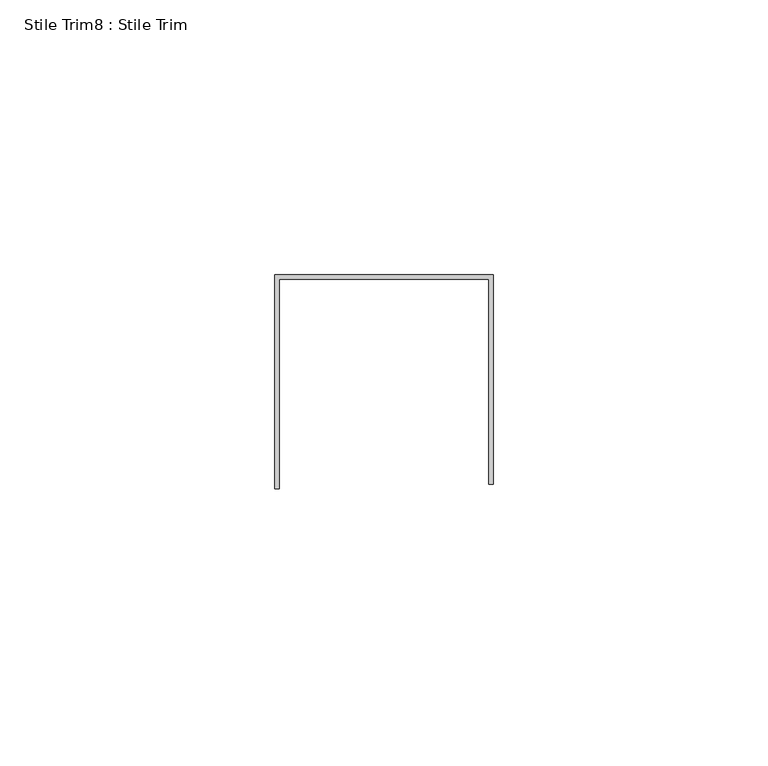
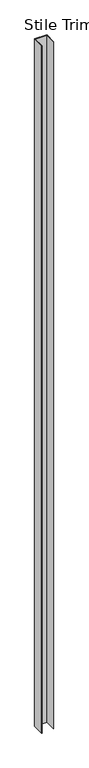
"""IFC4 building model written with IfcOpenShell, lengths in millimetres: proxy geometry, Stile Trim8 : Stile Trim."""

from ifc_helpers import new_model, si_unit, frame, origin, place, context, project, spatial, polyline, outline, extrude, source, transform, mapped, element, save


def stile_trim8_stile_trim_18cce888(model_context):
    return source(origin(), model_context, "Body", "SweptSolid", [
        extrude(outline(polyline([(587327.0060739, -535207.1289841), (587366.6808739, -535207.1289841), (587366.6808739, -535245.2289841), (587365.8934739, -535245.2289841), (587365.8934739, -535207.9163841), (587327.7934739, -535207.9163841), (587327.7934739, -535246.0163841), (587327.0060739, -535246.0163841), (587327.0060739, -535207.1289841)])), frame((0.0, 0.0, 50.8), z_axis=(0.0, 0.0, 1.0), x_axis=(1.0, 0.0, 0.0)), (0.0, 0.0, 1.0), 2350.3929688),
    ])


if __name__ == "__main__":
    model = new_model("IFC4")
    model_context = context("Model", 3, world=origin())
    ifc_project = project(units=[si_unit("LENGTHUNIT", "METRE", prefix="MILLI")], contexts=[model_context])
    site = spatial("IfcSite", under=ifc_project)
    building = spatial("IfcBuilding", under=site)
    placement = place(None, origin())
    stile_trim8_stile_trim_shape = stile_trim8_stile_trim_18cce888(model_context)
    element("IfcBuildingElementProxy", 1, Name="Stile Trim8 : Stile Trim", ObjectType="Stile Trim8 : Stile Trim", at=placement, inside=building, context=model_context, shape_type="MappedRepresentation", body=[
        mapped(stile_trim8_stile_trim_shape, transform((0.0, 0.0, 0.0), x_axis=(1.0, 0.0, 0.0), y_axis=(0.0, 1.0, 0.0), z_axis=(0.0, 0.0, 1.0))),
    ])
    save(model, "model.ifc")

# Revit data of these elements
# Element 1 (IfcBuildingElementProxy, "Stile Trim8 : Stile Trim")
#   Materials on its faces: "EDGE TRIM BY MTL PANEL MFR."
# Materials
#   "EDGE TRIM BY MTL PANEL MFR.": class "Generic", colour RGB 239 242 240, transparency 0, Cost = 0
